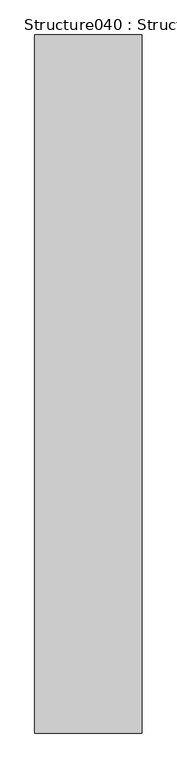
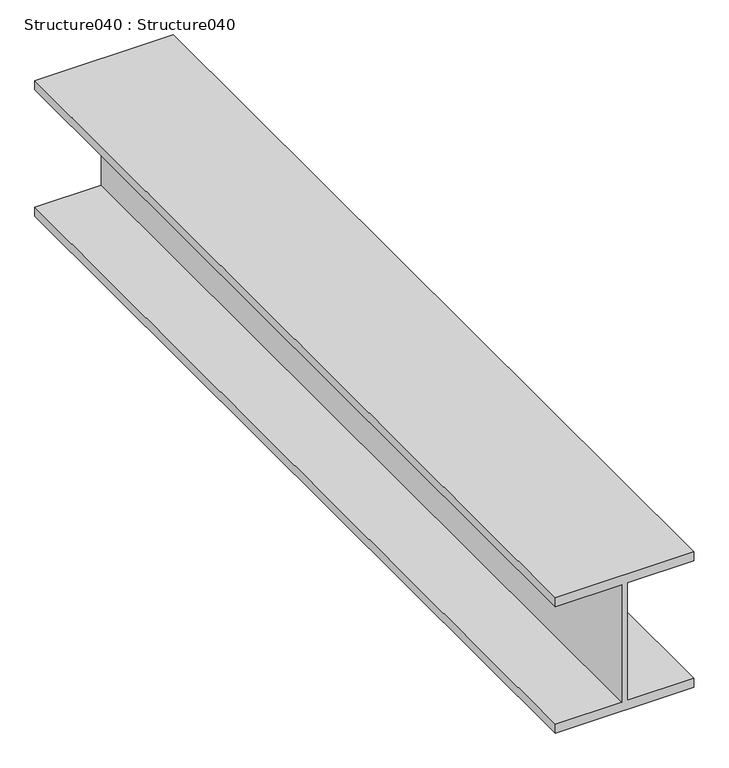
"""IFC4 building model written with IfcOpenShell, lengths in millimetres: proxy geometry, Structure040 : Structure040."""

from ifc_helpers import new_model, si_unit, frame, origin, place, context, project, spatial, polyline, outline, extrude, source, transform, mapped, element, save


def structure040_structure040_909150ff(model_context):
    return source(origin(), model_context, "Body", "SweptSolid", [
        extrude(outline(polyline([(40028.622, -4828.5743825), (39752.27, -4828.5743825), (39752.27, -4975.7038825), (39731.696, -4975.7038825), (39731.696, -4668.3638825), (39752.27, -4668.3638825), (39752.27, -4815.4933825), (40028.622, -4815.4933825), (40028.622, -4668.3638825), (40049.196, -4668.3638825), (40049.196, -4975.7038825), (40028.622, -4975.7038825), (40028.622, -4828.5743825)])), frame((0.0, -1052.8906574, 0.0), z_axis=(0.0, 1.0, 0.0), x_axis=(0.0, 0.0, 1.0)), (0.0, 0.0, 1.0), 2000.0),
    ])


if __name__ == "__main__":
    model = new_model("IFC4")
    model_context = context("Model", 3, world=origin())
    ifc_project = project(units=[si_unit("LENGTHUNIT", "METRE", prefix="MILLI")], contexts=[model_context])
    site = spatial("IfcSite", under=ifc_project)
    building = spatial("IfcBuilding", under=site)
    placement = place(None, origin())
    structure040_structure040_shape = structure040_structure040_909150ff(model_context)
    element("IfcBuildingElementProxy", 1, Name="Structure040 : Structure040", ObjectType="Structure040 : Structure040", at=placement, inside=building, context=model_context, shape_type="MappedRepresentation", body=[
        mapped(structure040_structure040_shape, transform((0.0, 0.0, 0.0), x_axis=(1.0, 0.0, 0.0), y_axis=(0.0, 1.0, 0.0), z_axis=(0.0, 0.0, 1.0))),
    ])
    save(model, "model.ifc")

# Revit data of these elements
# Type "Structure040 : Structure040"
#   NameOverride = "Structure040"
# Element 1 (IfcBuildingElementProxy, "Structure040 : Structure040")
#   Materials on its faces: "METAL STRUCTURE (SEE STRUCTURAL DWGS)"
# Materials
#   "METAL STRUCTURE (SEE STRUCTURAL DWGS)": class "Unassigned", colour RGB 128 128 128, transparency 0
